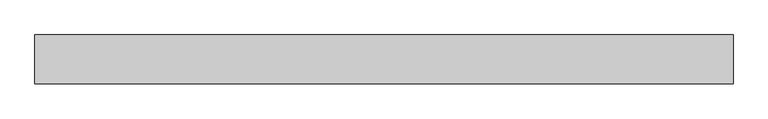
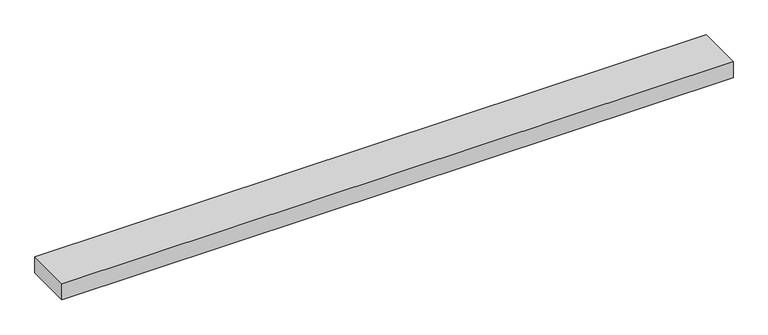
"""IFC4 building model written with IfcOpenShell, lengths in millimetres: proxy geometry, Blocking013 3005 : Blocking013 3005."""

from ifc_helpers import new_model, si_unit, frame, origin, place, context, project, spatial, polyline, outline, extrude, source, transform, mapped, element, save


def generic_models_ec4b54e7(model_context):
    return source(origin(), model_context, "Body", "SweptSolid", [
        extrude(outline(polyline([(3694.2883192, 10278.0250834), (3694.2883192, 10417.7250834), (5694.2883192, 10417.7250834), (5694.2883192, 10278.0250834), (3694.2883192, 10278.0250834)])), frame((0.0, 0.0, 43328.359375), z_axis=(0.0, 0.0, 1.0), x_axis=(1.0, 0.0, 0.0)), (0.0, 0.0, 1.0), 50.8),
    ])


if __name__ == "__main__":
    model = new_model("IFC4")
    model_context = context("Model", 3, world=origin())
    ifc_project = project(units=[si_unit("LENGTHUNIT", "METRE", prefix="MILLI")], contexts=[model_context])
    site = spatial("IfcSite", under=ifc_project)
    building = spatial("IfcBuilding", under=site)
    placement = place(None, origin())
    generic_models_shape = generic_models_ec4b54e7(model_context)
    element("IfcBuildingElementProxy", 1, Name="Blocking013 3005 : Blocking013 3005", ObjectType="Blocking013 3005 : Blocking013 3005", at=placement, inside=building, context=model_context, shape_type="MappedRepresentation", body=[
        mapped(generic_models_shape, transform((0.0, 0.0, 0.0), x_axis=(1.0, 0.0, 0.0), y_axis=(0.0, 1.0, 0.0), z_axis=(0.0, 0.0, 1.0))),
    ])
    save(model, "model.ifc")

# Revit data of these elements
# Type "Blocking013 3005 : Blocking013 3005"
#   NameOverride = "Blocking013"
# Element 1 (IfcBuildingElementProxy, "Blocking013 3005 : Blocking013 3005")
#   Materials on its faces: "WOOD BLOCKING AS REQUIRED"
# Materials
#   "WOOD BLOCKING AS REQUIRED": class "Unassigned", colour RGB 166 124 85, transparency 0, Cost = 0
